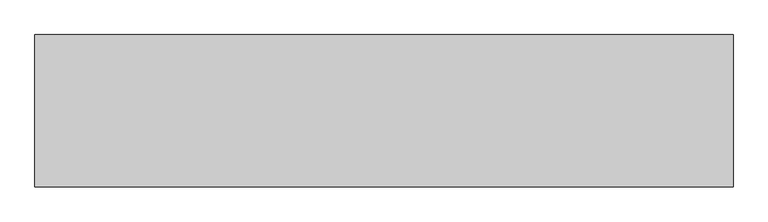
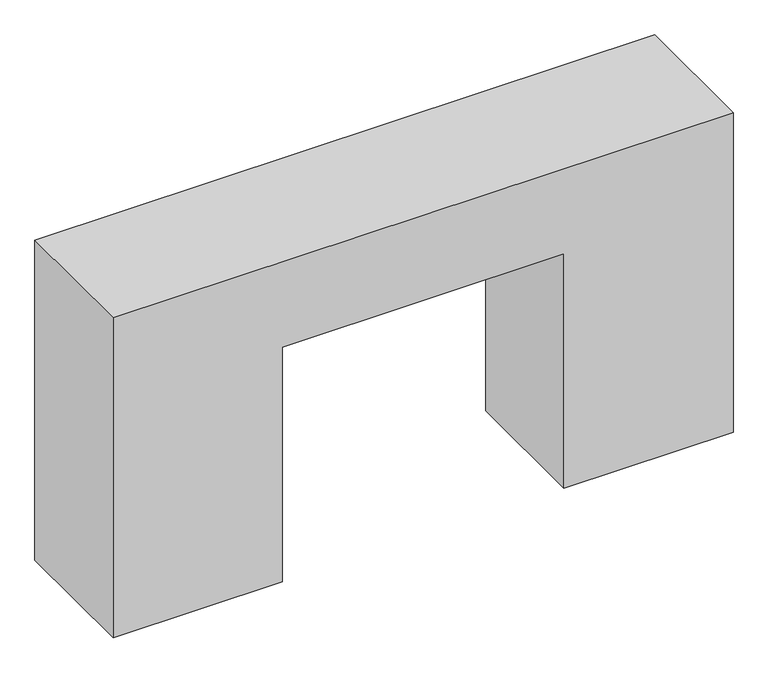
"""IFC4 building model written with IfcOpenShell, lengths in millimetres: proxy geometry, Generic Models 223:Generic Models 223:154187 : Generic Models 223:Generic Models 223:154187."""

from ifc_helpers import new_model, si_unit, frame, origin, place, context, project, spatial, polyline, outline, extrude, source, transform, mapped, element, save


def generic_models_4f30cc35(model_context):
    return source(origin(), model_context, "Body", "SweptSolid", [
        extrude(outline(polyline([(-304.8, 8531.1032131), (457.2, 8531.1032131), (457.2, 7134.103213), (-304.8, 7134.103213), (-304.8, 7515.103213), (254.0, 7515.103213), (254.0, 8150.1032131), (-304.8, 8150.1032131), (-304.8, 8531.1032131)])), frame((0.0, 4450.212823, 0.0), z_axis=(0.0, 1.0, 0.0), x_axis=(0.0, 0.0, 1.0)), (0.0, 0.0, 1.0), 304.8),
    ])


if __name__ == "__main__":
    model = new_model("IFC4")
    model_context = context("Model", 3, world=origin())
    ifc_project = project(units=[si_unit("LENGTHUNIT", "METRE", prefix="MILLI")], contexts=[model_context])
    site = spatial("IfcSite", under=ifc_project)
    building = spatial("IfcBuilding", under=site)
    placement = place(None, origin())
    generic_models_shape = generic_models_4f30cc35(model_context)
    element("IfcBuildingElementProxy", 1, Name="Generic Models 223:Generic Models 223:154187 : Generic Models 223:Generic Models 223:154187", ObjectType="Generic Models 223:Generic Models 223:154187 : Generic Models 223:Generic Models 223:154187", at=placement, inside=building, context=model_context, shape_type="MappedRepresentation", body=[
        mapped(generic_models_shape, transform((0.0, 0.0, 0.0), x_axis=(1.0, 0.0, 0.0), y_axis=(0.0, 1.0, 0.0), z_axis=(0.0, 0.0, 1.0))),
    ])
    save(model, "model.ifc")

# Revit data of these elements
# Type "Generic Models 223:Generic Models 223:154187 : Generic Models 223:Generic Models 223:154187"
#   NameOverride = "Generic Models 223:Generic Models 223:154187"
#   ObjectTypeOverride = "Generic Models 223:Generic Models 223"
#   Reference = "Generic Models 223"
#   Category = "Generic Models"
#   Tag = "154187"
# Element 1 (IfcBuildingElementProxy, "Generic Models 223:Generic Models 223:154187 : Generic Models 223:Generic Models 223:154187")
#   Materials on its faces: "_CONCRETE SLAB W/ WIRE MESH (SEE STRUCT. DWGS) 20583"
# Materials
#   "_CONCRETE SLAB W/ WIRE MESH (SEE STRUCT. DWGS) 20583": class "Unassigned", colour RGB 191 191 191, transparency 0
